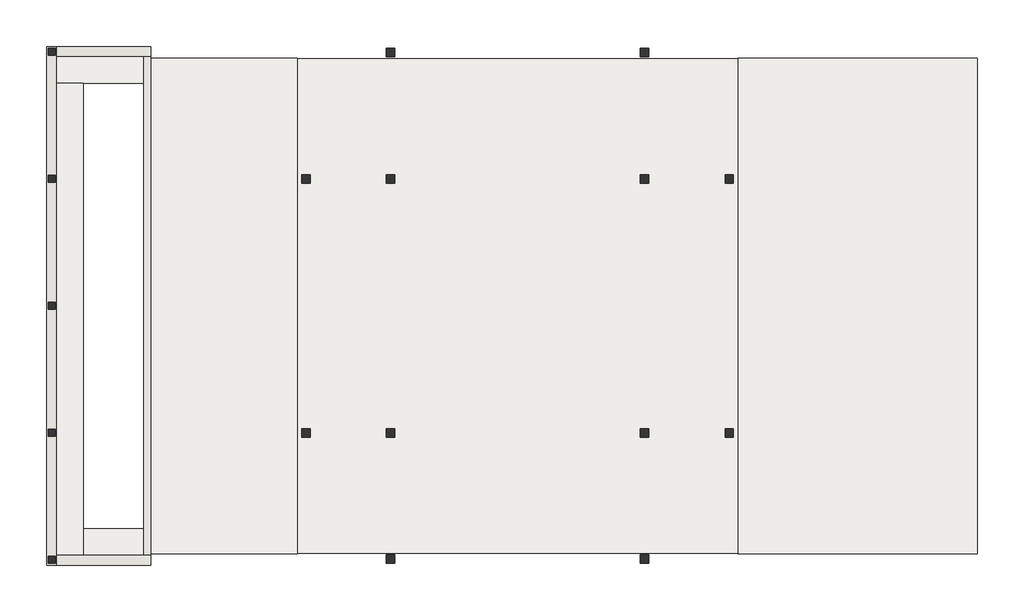
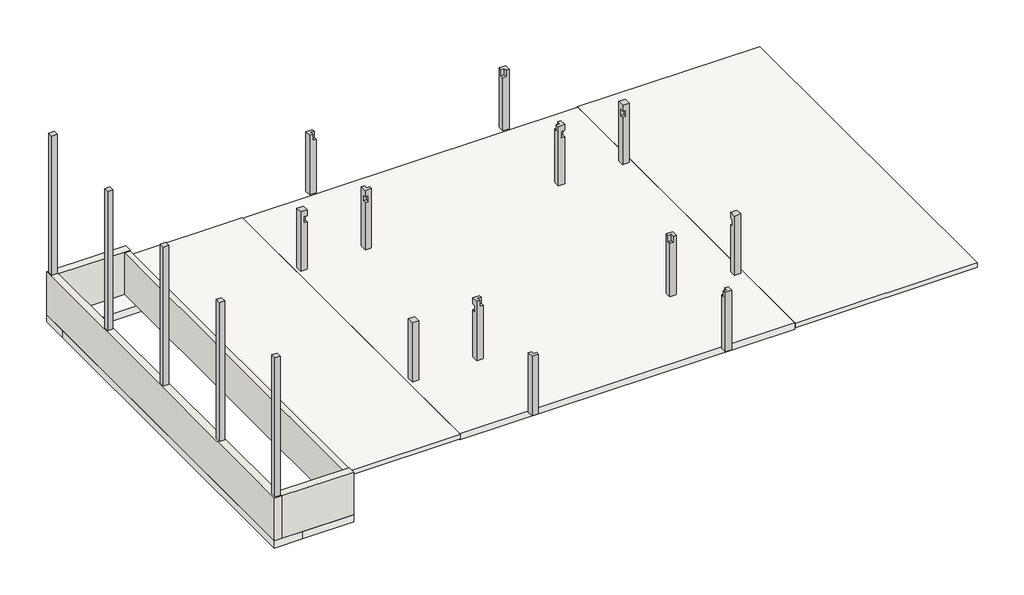
# One storey: 17 columns, 4 walls, 3 footings, 3 slabs.
"""IFC4 building model written with IfcOpenShell, lengths in millimetres."""

import ifcopenshell
import ifcopenshell.guid

model = None  # the IFC model being written
_history = None  # IfcOwnerHistory: only IFC2X3 demands one
_inside = {}  # id of a spatial element -> (the spatial element, [elements in it])
_under = {}  # id of a project, library or spatial element -> (it, [spatial elements below it])
_declared = {}  # id of a project -> (the project, [libraries it declares])
_typed = {}  # id of a type object -> (the type object, [elements of that type])
_made_of = {}  # id of a material, layer set ... -> (it, [elements and type objects made of it])


def new_model(schema):
    """Start an empty IFC model of exactly this schema.

    Asked for "IFC4X3", IfcOpenShell would pick the latest addendum, in which some entities
    have other attributes; the version numbers below select the first issue.
    IFC2X3 requires an IfcOwnerHistory on every rooted entity: one is made here for all.
    """
    global model, _history
    if schema == "IFC4X3":
        model = ifcopenshell.file(schema_version=(4, 3, 0, 0))
    else:
        model = ifcopenshell.file(schema=schema)
    _inside.clear()
    _under.clear()
    _declared.clear()
    _typed.clear()
    _made_of.clear()
    _history = None
    if model.schema == "IFC2X3":
        org = make("IfcOrganization", Name="unknown")
        user = make(
            "IfcPersonAndOrganization",
            ThePerson=make("IfcPerson", FamilyName="unknown"),
            TheOrganization=org,
        )
        app = make(
            "IfcApplication",
            ApplicationDeveloper=org,
            Version="unknown",
            ApplicationFullName="unknown",
            ApplicationIdentifier="unknown",
        )
        _history = make(
            "IfcOwnerHistory",
            OwningUser=user,
            OwningApplication=app,
            ChangeAction="ADDED",
            CreationDate=0,
        )
    return model


def make(cls, **values):
    """One entity of the class cls with the attributes given. An attribute that is None is left unset."""
    return model.create_entity(
        cls, **{name: value for name, value in values.items() if value is not None}
    )


def rooted(cls, **values):
    """An entity with a GlobalId (a new one), such as an element, a storey or a relation."""
    return make(cls, GlobalId=ifcopenshell.guid.new(), OwnerHistory=_history, **values)


def si_unit(unit_type, name, prefix=None):
    """IfcSIUnit, for example si_unit("LENGTHUNIT", "METRE", prefix="MILLI")."""
    return make("IfcSIUnit", UnitType=unit_type, Prefix=prefix, Name=name)


def assignment(units):
    """IfcUnitAssignment: the units of a project."""
    return None if units is None else make("IfcUnitAssignment", Units=units)


def point(xyz):
    """IfcCartesianPoint."""
    return None if xyz is None else make("IfcCartesianPoint", Coordinates=xyz)


def direction(xyz):
    """IfcDirection."""
    return None if xyz is None else make("IfcDirection", DirectionRatios=xyz)


def frame(location, z_axis=None, x_axis=None):
    """IfcAxis2Placement3D, a coordinate frame: its origin and axes. An axis left out is left unset."""
    return make(
        "IfcAxis2Placement3D",
        Location=point(location),
        Axis=direction(z_axis),
        RefDirection=direction(x_axis),
    )


def origin():
    """The frame at (0, 0, 0) with its axes left unset."""
    return frame((0.0, 0.0, 0.0))


def origin_with_axes():
    """The frame at (0, 0, 0) with the z axis (0, 0, 1) and the x axis (1, 0, 0) written out."""
    return frame((0.0, 0.0, 0.0), z_axis=(0.0, 0.0, 1.0), x_axis=(1.0, 0.0, 0.0))


def place(relative_to, where):
    """IfcLocalPlacement: puts the frame where relative to a parent placement (None: the world)."""
    return make(
        "IfcLocalPlacement", PlacementRelTo=relative_to, RelativePlacement=where
    )


def context(
    kind, dimensions, precision=None, world=None, true_north=None, identifier=None
):
    """IfcGeometricRepresentationContext, for example the 3D "Model" context."""
    return make(
        "IfcGeometricRepresentationContext",
        ContextIdentifier=identifier,
        ContextType=kind,
        CoordinateSpaceDimension=dimensions,
        Precision=precision,
        WorldCoordinateSystem=world,
        TrueNorth=true_north,
    )


def project(units=None, contexts=None):
    """IfcProject with its units and contexts."""
    return rooted(
        "IfcProject",
        Name="project",
        RepresentationContexts=contexts,
        UnitsInContext=assignment(units),
    )


def spatial(cls, under=None, at=None, **own):
    """A site, building, storey or space (cls), placed at a placement, below another one or the project."""
    s = rooted(cls, ObjectPlacement=at, **own)
    if under is not None:
        _under.setdefault(under.id(), (under, []))[1].append(s)
    return s


def polyline(points):
    """IfcPolyline through the points."""
    return make("IfcPolyline", Points=[point(p) for p in points])


def outline(outer, holes=None, kind="AREA"):
    """IfcArbitraryClosedProfileDef: a profile drawn as a closed curve; with holes, ...WithVoids."""
    if holes is None:
        return make("IfcArbitraryClosedProfileDef", ProfileType=kind, OuterCurve=outer)
    return make(
        "IfcArbitraryProfileDefWithVoids",
        ProfileType=kind,
        OuterCurve=outer,
        InnerCurves=holes,
    )


def extrude(swept, where, along, depth):
    """IfcExtrudedAreaSolid: the profile swept, set in the frame where, extruded along a direction by depth."""
    return make(
        "IfcExtrudedAreaSolid",
        SweptArea=swept,
        Position=where,
        ExtrudedDirection=direction(along),
        Depth=depth,
    )


def faces_of(points, faces, orient=None, outer=None):
    """IfcFace entities. A face is a list of loops; a loop is a list of indices into points, from 0.

    orient and outer hold one flag for each loop. By default every Orientation is true, the
    first loop of a face is its IfcFaceOuterBound and the others are IfcFaceBound.
    """
    made = []
    for i, loops in enumerate(faces):
        bounds = []
        for j, loop in enumerate(loops):
            is_outer = j == 0 if outer is None else outer[i][j]
            bounds.append(
                make(
                    "IfcFaceOuterBound" if is_outer else "IfcFaceBound",
                    Bound=make("IfcPolyLoop", Polygon=[points[k] for k in loop]),
                    Orientation=True if orient is None else orient[i][j],
                )
            )
        made.append(make("IfcFace", Bounds=bounds))
    return made


def faceted_brep(points, faces, orient=None, outer=None, voids=None):
    """IfcFacetedBrep: a solid bounded by flat faces; with voids (closed shells), ...WithVoids."""
    shared = [point(p) for p in points]
    hull = make("IfcClosedShell", CfsFaces=faces_of(shared, faces, orient, outer))
    if voids is None:
        return make("IfcFacetedBrep", Outer=hull)
    return make(
        "IfcFacetedBrepWithVoids",
        Outer=hull,
        Voids=[
            make(cls, CfsFaces=faces_of(shared, fs, o, b)) for cls, fs, o, b in voids
        ],
    )


def shape(context_of_items, identifier, shape_type, items):
    """IfcShapeRepresentation: the items that make up one representation, for example the "Body"."""
    return make(
        "IfcShapeRepresentation",
        ContextOfItems=context_of_items,
        RepresentationIdentifier=identifier,
        RepresentationType=shape_type,
        Items=items,
    )


def made_of(thing, what):
    """Note that an element or type object is made of a material, layer set ...; save() writes the relation."""
    if what is not None:
        _made_of.setdefault(what.id(), (what, []))[1].append(thing)
    return thing


def element(
    cls,
    number,
    at=None,
    inside=None,
    cuts=None,
    type_object=None,
    material=None,
    context=None,
    identifier="Body",
    shape_type=None,
    held_by="IfcProductDefinitionShape",
    body=None,
    shapes=None,
    **own,
):
    """One element of the class cls, such as IfcWall. Its Tag is "e" and its number.

    at: its placement. inside: the storey or other place that contains it. cuts: it is an
    opening in that element (IfcRelVoidsElement). A single representation is given by context,
    identifier, shape_type and body (its items); several are given by shapes. held_by: the class
    of the entity that holds the representations. save() writes the other relations.
    """
    e = rooted(cls, Tag="e%d" % number, ObjectPlacement=at, **own)
    if body is not None:
        shapes = [shape(context, identifier, shape_type, body)]
    if shapes is not None:
        e.Representation = make(held_by, Representations=shapes)
    if inside is not None:
        _inside.setdefault(inside.id(), (inside, []))[1].append(e)
    if cuts is not None:
        rooted(
            "IfcRelVoidsElement", RelatingBuildingElement=cuts, RelatedOpeningElement=e
        )
    if type_object is not None:
        _typed.setdefault(type_object.id(), (type_object, []))[1].append(e)
    return made_of(e, material)


def aggregate(whole, parts):
    """IfcRelAggregates: a whole, such as a stair, and the parts it consists of."""
    return rooted("IfcRelAggregates", RelatingObject=whole, RelatedObjects=parts)


def save(model, path):
    """Write the relations noted so far, then the file.

    IfcRelAggregates (storeys below a building ...), IfcRelContainedInSpatialStructure (elements
    in a storey), IfcRelDefinesByType, IfcRelAssociatesMaterial and IfcRelDeclares: one each for
    every whole, place, type object, material and project.
    """
    for whole, parts in _under.values():
        aggregate(whole, parts)
    for where, things in _inside.values():
        rooted(
            "IfcRelContainedInSpatialStructure",
            RelatedElements=things,
            RelatingStructure=where,
        )
    for kind, things in _typed.values():
        rooted("IfcRelDefinesByType", RelatedObjects=things, RelatingType=kind)
    for what, things in _made_of.values():
        rooted("IfcRelAssociatesMaterial", RelatedObjects=things, RelatingMaterial=what)
    for by, libraries in _declared.values():
        rooted("IfcRelDeclares", RelatingContext=by, RelatedDefinitions=libraries)
    model.write(path)


model = new_model("IFC4")

# Units and contexts
model_context = context("Model", 3, world=origin())
ifc_project = project(units=[si_unit("LENGTHUNIT", "METRE", prefix="MILLI")], contexts=[model_context])

# Site, building, storey
site = spatial("IfcSite", under=ifc_project)
building = spatial("IfcBuilding", under=site)
storey = spatial("IfcBuildingStorey", under=building, Name="E-ACCESO", Elevation=0.0)

# Columns
placement = place(None, origin())
element("IfcColumn", 1, ObjectType="Hormigón-Cuadrado-Pilar : PILAR 25X25", at=placement, inside=storey, context=model_context, shape_type="SweptSolid", body=[
    extrude(outline(polyline([(-32875.0, -4375.0), (-32875.0, -4625.0), (-33125.0, -4625.0), (-33125.0, -4375.0), (-32875.0, -4375.0)])), origin_with_axes(), (0.0, 0.0, 1.0), 6850.0),
])
element("IfcColumn", 2, ObjectType="Hormigón-Cuadrado-Pilar : PILAR 25X25", at=placement, inside=storey, context=model_context, shape_type="SweptSolid", body=[
    extrude(outline(polyline([(-32875.0, -8875.0), (-32875.0, -9125.0), (-33125.0, -9125.0), (-33125.0, -8875.0), (-32875.0, -8875.0)])), origin_with_axes(), (0.0, 0.0, 1.0), 6850.0),
])
element("IfcColumn", 3, ObjectType="Hormigón-Cuadrado-Pilar : PILAR 25X25", at=placement, inside=storey, context=model_context, shape_type="SweptSolid", body=[
    extrude(outline(polyline([(-32875.0, -13375.0), (-32875.0, -13625.0), (-33125.0, -13625.0), (-33125.0, -13375.0), (-32875.0, -13375.0)])), origin_with_axes(), (0.0, 0.0, 1.0), 6850.0),
])
element("IfcColumn", 4, ObjectType="Hormigón-Cuadrado-Pilar : PILAR 25X25", at=placement, inside=storey, context=model_context, shape_type="SweptSolid", body=[
    extrude(outline(polyline([(-32875.0, -17875.0), (-32875.0, -18125.0), (-33125.0, -18125.0), (-33125.0, -17875.0), (-32875.0, -17875.0)])), origin_with_axes(), (0.0, 0.0, 1.0), 6850.0),
])
element("IfcColumn", 5, ObjectType="Hormigón-Cuadrado-Pilar : PILAR 25X25", at=placement, inside=storey, context=model_context, shape_type="SweptSolid", body=[
    extrude(outline(polyline([(-32875.0, 125.0), (-32875.0, -125.0), (-33125.0, -125.0), (-33125.0, 125.0), (-32875.0, 125.0)])), origin_with_axes(), (0.0, 0.0, 1.0), 6850.0),
])
element("IfcColumn", 6, ObjectType="Hormigón-Cuadrado-Pilar : PILAR 30X30", at=placement, inside=storey, context=model_context, shape_type="Brep", body=[
    faceted_brep([(-23850.0, -4350.0, -200.0), (-23850.0, -4650.0, -200.0), (-24150.0, -4650.0, -200.0), (-24150.0, -4350.0, -200.0), (-23850.0, -4350.0, 2730.0), (-23850.0, -4650.0, 2730.0), (-23850.0, -4650.0, 2430.0), (-23850.0, -4500.0, 2430.0), (-23850.0, -4500.0, 2130.0), (-23850.0, -4650.0, 2130.0), (-24000.0, -4650.0, 2130.0), (-24000.0, -4650.0, 2430.0), (-24150.0, -4650.0, 2730.0), (-24150.0, -4350.0, 2730.0), (-24000.0, -4500.0, 2130.0), (-24000.0, -4500.0, 2430.0)], [[[0, 1, 2, 3]], [[1, 0, 4, 5, 6, 7, 8, 9]], [[2, 1, 9, 10, 11, 6, 5, 12]], [[3, 2, 12, 13]], [[0, 3, 13, 4]], [[5, 4, 13, 12]], [[8, 14, 10, 9]], [[11, 15, 7, 6]], [[14, 15, 11, 10]], [[15, 14, 8, 7]]]),
])
element("IfcColumn", 7, ObjectType="Hormigón-Cuadrado-Pilar : PILAR 30X30", at=placement, inside=storey, context=model_context, shape_type="Brep", body=[
    faceted_brep([(-20850.0, -4350.0, -200.0), (-20850.0, -4650.0, -200.0), (-21150.0, -4650.0, -200.0), (-21150.0, -4350.0, -200.0), (-20850.0, -4350.0, 2430.0), (-20850.0, -4500.0, 2430.0), (-20850.0, -4500.0, 2730.0), (-20850.0, -4650.0, 2730.0), (-21150.0, -4650.0, 2730.0), (-21150.0, -4650.0, 2430.0), (-21000.0, -4650.0, 2430.0), (-21000.0, -4650.0, 2130.0), (-21150.0, -4650.0, 2130.0), (-21150.0, -4500.0, 2130.0), (-21150.0, -4500.0, 2430.0), (-21150.0, -4350.0, 2730.0), (-21000.0, -4350.0, 2730.0), (-21000.0, -4350.0, 2430.0), (-21000.0, -4500.0, 2730.0), (-21000.0, -4500.0, 2430.0), (-21000.0, -4500.0, 2130.0), (-21000.0, -4500.0, 2430.0)], [[[0, 1, 2, 3]], [[1, 0, 4, 5, 6, 7]], [[2, 1, 7, 8, 9, 10, 11, 12]], [[3, 2, 12, 13, 14, 9, 8, 15]], [[0, 3, 15, 16, 17, 4]], [[8, 7, 6, 18, 16, 15]], [[19, 5, 4, 17]], [[18, 19, 17, 16]], [[19, 18, 6, 5]], [[20, 13, 12, 11]], [[21, 10, 9, 14]], [[21, 20, 11, 10]], [[20, 21, 14, 13]]]),
])
element("IfcColumn", 8, ObjectType="Hormigón-Cuadrado-Pilar : PILAR 30X30", at=placement, inside=storey, context=model_context, shape_type="Brep", body=[
    faceted_brep([(-11850.0, -4350.0, -200.0), (-11850.0, -4650.0, -200.0), (-12150.0, -4650.0, -200.0), (-12150.0, -4350.0, -200.0), (-11850.0, -4350.0, 2730.0), (-11850.0, -4650.0, 2730.0), (-11850.0, -4650.0, 2430.0), (-11850.0, -4500.0, 2430.0), (-11850.0, -4500.0, 2130.0), (-11850.0, -4650.0, 2130.0), (-12000.0, -4650.0, 2130.0), (-12000.0, -4650.0, 2430.0), (-12150.0, -4650.0, 2730.0), (-12150.0, -4500.0, 2730.0), (-12150.0, -4500.0, 2430.0), (-12150.0, -4350.0, 2430.0), (-12000.0, -4350.0, 2430.0), (-12000.0, -4350.0, 2730.0), (-12000.0, -4500.0, 2730.0), (-12000.0, -4500.0, 2430.0), (-12000.0, -4500.0, 2130.0), (-12000.0, -4500.0, 2430.0)], [[[0, 1, 2, 3]], [[1, 0, 4, 5, 6, 7, 8, 9]], [[2, 1, 9, 10, 11, 6, 5, 12]], [[3, 2, 12, 13, 14, 15]], [[0, 3, 15, 16, 17, 4]], [[5, 4, 17, 18, 13, 12]], [[14, 19, 16, 15]], [[19, 18, 17, 16]], [[18, 19, 14, 13]], [[8, 20, 10, 9]], [[11, 21, 7, 6]], [[20, 21, 11, 10]], [[21, 20, 8, 7]]]),
])
element("IfcColumn", 9, ObjectType="Hormigón-Cuadrado-Pilar : PILAR 30X30", at=placement, inside=storey, context=model_context, shape_type="Brep", body=[
    faceted_brep([(-8850.0, -4350.0, -200.0), (-8850.0, -4650.0, -200.0), (-9150.0, -4650.0, -200.0), (-9150.0, -4350.0, -200.0), (-8850.0, -4350.0, 2730.0), (-8850.0, -4650.0, 2730.0), (-9150.0, -4650.0, 2730.0), (-9150.0, -4650.0, 2430.0), (-9000.0, -4650.0, 2430.0), (-9000.0, -4650.0, 2130.0), (-9150.0, -4650.0, 2130.0), (-9150.0, -4500.0, 2130.0), (-9150.0, -4500.0, 2430.0), (-9150.0, -4350.0, 2730.0), (-9000.0, -4500.0, 2130.0), (-9000.0, -4500.0, 2430.0)], [[[0, 1, 2, 3]], [[1, 0, 4, 5]], [[2, 1, 5, 6, 7, 8, 9, 10]], [[3, 2, 10, 11, 12, 7, 6, 13]], [[0, 3, 13, 4]], [[5, 4, 13, 6]], [[14, 11, 10, 9]], [[15, 8, 7, 12]], [[15, 14, 9, 8]], [[14, 15, 12, 11]]]),
])
element("IfcColumn", 10, ObjectType="Hormigón-Cuadrado-Pilar : PILAR 30X30", at=placement, inside=storey, context=model_context, shape_type="Brep", body=[
    faceted_brep([(-8850.0, -13350.0, -200.0), (-8850.0, -13650.0, -200.0), (-9150.0, -13650.0, -200.0), (-9150.0, -13350.0, -200.0), (-8850.0, -13350.0, 2730.0), (-8850.0, -13650.0, 2730.0), (-9150.0, -13650.0, 2730.0), (-9150.0, -13350.0, 2730.0), (-9150.0, -13350.0, 2430.0), (-9150.0, -13500.0, 2430.0), (-9150.0, -13500.0, 2130.0), (-9150.0, -13350.0, 2130.0), (-9000.0, -13350.0, 2130.0), (-9000.0, -13350.0, 2430.0), (-9000.0, -13500.0, 2130.0), (-9000.0, -13500.0, 2430.0)], [[[0, 1, 2, 3]], [[1, 0, 4, 5]], [[2, 1, 5, 6]], [[3, 2, 6, 7, 8, 9, 10, 11]], [[0, 3, 11, 12, 13, 8, 7, 4]], [[5, 4, 7, 6]], [[10, 14, 12, 11]], [[13, 15, 9, 8]], [[14, 15, 13, 12]], [[15, 14, 10, 9]]]),
])
element("IfcColumn", 11, ObjectType="Hormigón-Cuadrado-Pilar : PILAR 30X30", at=placement, inside=storey, context=model_context, shape_type="Brep", body=[
    faceted_brep([(-11850.0, -13350.0, -200.0), (-11850.0, -13650.0, -200.0), (-12150.0, -13650.0, -200.0), (-12150.0, -13350.0, -200.0), (-11850.0, -13350.0, 2130.0), (-11850.0, -13500.0, 2130.0), (-11850.0, -13500.0, 2430.0), (-11850.0, -13350.0, 2430.0), (-11850.0, -13350.0, 2730.0), (-11850.0, -13650.0, 2730.0), (-12000.0, -13650.0, 2730.0), (-12000.0, -13650.0, 2430.0), (-12150.0, -13650.0, 2430.0), (-12150.0, -13500.0, 2430.0), (-12150.0, -13500.0, 2730.0), (-12150.0, -13350.0, 2730.0), (-12000.0, -13350.0, 2430.0), (-12000.0, -13350.0, 2130.0), (-12000.0, -13500.0, 2730.0), (-12000.0, -13500.0, 2430.0), (-12000.0, -13500.0, 2130.0), (-12000.0, -13500.0, 2430.0)], [[[0, 1, 2, 3]], [[1, 0, 4, 5, 6, 7, 8, 9]], [[2, 1, 9, 10, 11, 12]], [[3, 2, 12, 13, 14, 15]], [[0, 3, 15, 8, 7, 16, 17, 4]], [[9, 8, 15, 14, 18, 10]], [[19, 13, 12, 11]], [[18, 19, 11, 10]], [[19, 18, 14, 13]], [[17, 20, 5, 4]], [[6, 21, 16, 7]], [[20, 21, 6, 5]], [[21, 20, 17, 16]]]),
])
element("IfcColumn", 12, ObjectType="Hormigón-Cuadrado-Pilar : PILAR 30X30", at=placement, inside=storey, context=model_context, shape_type="Brep", body=[
    faceted_brep([(-20850.0, -13350.0, -200.0), (-20850.0, -13650.0, -200.0), (-21150.0, -13650.0, -200.0), (-21150.0, -13350.0, -200.0), (-20850.0, -13350.0, 2730.0), (-20850.0, -13500.0, 2730.0), (-20850.0, -13500.0, 2430.0), (-20850.0, -13650.0, 2430.0), (-21000.0, -13650.0, 2430.0), (-21000.0, -13650.0, 2730.0), (-21150.0, -13650.0, 2730.0), (-21150.0, -13350.0, 2730.0), (-21150.0, -13350.0, 2430.0), (-21150.0, -13500.0, 2430.0), (-21150.0, -13500.0, 2130.0), (-21150.0, -13350.0, 2130.0), (-21000.0, -13350.0, 2130.0), (-21000.0, -13350.0, 2430.0), (-21000.0, -13500.0, 2730.0), (-21000.0, -13500.0, 2430.0), (-21000.0, -13500.0, 2130.0), (-21000.0, -13500.0, 2430.0)], [[[0, 1, 2, 3]], [[1, 0, 4, 5, 6, 7]], [[2, 1, 7, 8, 9, 10]], [[3, 2, 10, 11, 12, 13, 14, 15]], [[0, 3, 15, 16, 17, 12, 11, 4]], [[11, 10, 9, 18, 5, 4]], [[6, 19, 8, 7]], [[19, 18, 9, 8]], [[18, 19, 6, 5]], [[14, 20, 16, 15]], [[17, 21, 13, 12]], [[20, 21, 17, 16]], [[21, 20, 14, 13]]]),
])
element("IfcColumn", 13, ObjectType="Hormigón-Cuadrado-Pilar : PILAR 30X30", at=placement, inside=storey, context=model_context, shape_type="Brep", body=[
    faceted_brep([(-23850.0, -13350.0, -200.0), (-23850.0, -13650.0, -200.0), (-24150.0, -13650.0, -200.0), (-24150.0, -13350.0, -200.0), (-23850.0, -13350.0, 2130.0), (-23850.0, -13500.0, 2130.0), (-23850.0, -13500.0, 2430.0), (-23850.0, -13350.0, 2430.0), (-23850.0, -13350.0, 2730.0), (-23850.0, -13650.0, 2730.0), (-24150.0, -13650.0, 2730.0), (-24150.0, -13350.0, 2730.0), (-24000.0, -13350.0, 2430.0), (-24000.0, -13350.0, 2130.0), (-24000.0, -13500.0, 2130.0), (-24000.0, -13500.0, 2430.0)], [[[0, 1, 2, 3]], [[1, 0, 4, 5, 6, 7, 8, 9]], [[2, 1, 9, 10]], [[3, 2, 10, 11]], [[0, 3, 11, 8, 7, 12, 13, 4]], [[9, 8, 11, 10]], [[13, 14, 5, 4]], [[6, 15, 12, 7]], [[14, 15, 6, 5]], [[15, 14, 13, 12]]]),
])
element("IfcColumn", 14, ObjectType="Hormigón-Cuadrado-Pilar : PILAR 30X30", at=placement, inside=storey, context=model_context, shape_type="Brep", body=[
    faceted_brep([(-20850.0, -17825.0, -200.0), (-20850.0, -18125.0, -200.0), (-21150.0, -18125.0, -200.0), (-21150.0, -17825.0, -200.0), (-20850.0, -17825.0, 2430.0), (-20850.0, -17975.0, 2430.0), (-20850.0, -17975.0, 2730.0), (-20850.0, -18125.0, 2730.0), (-21150.0, -18125.0, 2730.0), (-21150.0, -17825.0, 2730.0), (-21000.0, -17825.0, 2730.0), (-21000.0, -17825.0, 2430.0), (-21000.0, -17975.0, 2730.0), (-21000.0, -17975.0, 2430.0)], [[[0, 1, 2, 3]], [[1, 0, 4, 5, 6, 7]], [[2, 1, 7, 8]], [[3, 2, 8, 9]], [[0, 3, 9, 10, 11, 4]], [[8, 7, 6, 12, 10, 9]], [[11, 13, 5, 4]], [[13, 12, 6, 5]], [[12, 13, 11, 10]]]),
])
element("IfcColumn", 15, ObjectType="Hormigón-Cuadrado-Pilar : PILAR 30X30", at=placement, inside=storey, context=model_context, shape_type="Brep", body=[
    faceted_brep([(-20850.0, 125.0, -200.0), (-20850.0, -175.0, -200.0), (-21150.0, -175.0, -200.0), (-21150.0, 125.0, -200.0), (-20850.0, 125.0, 2730.0), (-20850.0, -25.0, 2730.0), (-20850.0, -25.0, 2430.0), (-20850.0, -175.0, 2430.0), (-21150.0, 125.0, 2730.0), (-21150.0, -175.0, 2730.0), (-21000.0, -175.0, 2430.0), (-21000.0, -175.0, 2730.0), (-21000.0, -25.0, 2730.0), (-21000.0, -25.0, 2430.0)], [[[0, 1, 2, 3]], [[1, 0, 4, 5, 6, 7]], [[0, 3, 8, 4]], [[3, 2, 9, 8]], [[2, 1, 7, 10, 11, 9]], [[4, 8, 9, 11, 12, 5]], [[6, 13, 10, 7]], [[13, 12, 11, 10]], [[12, 13, 6, 5]]]),
])
element("IfcColumn", 16, ObjectType="Hormigón-Cuadrado-Pilar : PILAR 30X30", at=placement, inside=storey, context=model_context, shape_type="Brep", body=[
    faceted_brep([(-12150.0, -18125.0, -200.0), (-12150.0, -17825.0, -200.0), (-11850.0, -17825.0, -200.0), (-11850.0, -18125.0, -200.0), (-12150.0, -18125.0, 2730.0), (-12150.0, -17975.0, 2730.0), (-12150.0, -17975.0, 2430.0), (-12150.0, -17825.0, 2430.0), (-11850.0, -18125.0, 2730.0), (-11850.0, -17825.0, 2730.0), (-12000.0, -17825.0, 2430.0), (-12000.0, -17825.0, 2730.0), (-12000.0, -17975.0, 2730.0), (-12000.0, -17975.0, 2430.0)], [[[0, 1, 2, 3]], [[1, 0, 4, 5, 6, 7]], [[0, 3, 8, 4]], [[3, 2, 9, 8]], [[2, 1, 7, 10, 11, 9]], [[4, 8, 9, 11, 12, 5]], [[6, 13, 10, 7]], [[13, 12, 11, 10]], [[12, 13, 6, 5]]]),
])
element("IfcColumn", 17, ObjectType="Hormigón-Cuadrado-Pilar : PILAR 30X30", at=placement, inside=storey, context=model_context, shape_type="Brep", body=[
    faceted_brep([(-12150.0, -175.0, -200.0), (-12150.0, 125.0, -200.0), (-11850.0, 125.0, -200.0), (-11850.0, -175.0, -200.0), (-12150.0, -175.0, 2430.0), (-12150.0, -25.0, 2430.0), (-12150.0, -25.0, 2730.0), (-12150.0, 125.0, 2730.0), (-11850.0, 125.0, 2730.0), (-11850.0, -175.0, 2730.0), (-12000.0, -175.0, 2730.0), (-12000.0, -175.0, 2430.0), (-12000.0, -25.0, 2730.0), (-12000.0, -25.0, 2430.0)], [[[0, 1, 2, 3]], [[1, 0, 4, 5, 6, 7]], [[2, 1, 7, 8]], [[3, 2, 8, 9]], [[0, 3, 9, 10, 11, 4]], [[8, 7, 6, 12, 10, 9]], [[11, 13, 5, 4]], [[13, 12, 6, 5]], [[12, 13, 11, 10]]]),
])

# Footings
element("IfcFooting", 18, ObjectType="CIMENT MURO PISCINA_PABLO", at=placement, inside=storey, context=model_context, shape_type="Brep", body=[
    faceted_brep([(-31890.0, -18190.0, -2100.0), (-31890.0, -16890.0, -2100.0), (-31890.0, -1110.0, -2100.0), (-33190.0, -1110.0, -2100.0), (-33190.0, -18190.0, -2100.0), (-32840.0, -18190.0, -2100.0), (-33190.0, -18190.0, -2450.0), (-33190.0, -1110.0, -2450.0), (-31890.0, -18190.0, -2450.0), (-31890.0, -1110.0, -2450.0), (-31890.0, -16890.0, -2450.0)], [[[0, 1, 2, 3, 4, 5]], [[6, 4, 3, 7]], [[8, 6, 7, 9, 10]], [[0, 8, 10, 9, 2, 1]], [[3, 2, 9, 7]], [[0, 5, 4, 6, 8]]]),
])
element("IfcFooting", 19, ObjectType="CIMENT MURO PISCINA_PABLO", at=placement, inside=storey, context=model_context, shape_type="Brep", body=[
    faceted_brep([(-29500.0, 190.0, -2100.0), (-29500.0, -1110.0, -2100.0), (-29500.0, -1110.0, -2450.0), (-29500.0, 190.0, -2450.0), (-33190.0, -1110.0, -2100.0), (-31890.0, -1110.0, -2100.0), (-33190.0, 190.0, -2100.0), (-33190.0, 190.0, -2450.0), (-33190.0, -1110.0, -2450.0), (-31890.0, -1110.0, -2450.0)], [[[0, 1, 2, 3]], [[4, 5, 1, 0, 6]], [[7, 6, 0, 3]], [[8, 7, 3, 2, 9]], [[4, 8, 9, 2, 1, 5]], [[4, 6, 7, 8]]]),
])
element("IfcFooting", 20, ObjectType="CIMENT MURO PISCINA_PABLO", at=placement, inside=storey, context=model_context, shape_type="SweptSolid", body=[
    extrude(outline(polyline([(-29500.0, -16890.0), (-29500.0, -18190.0), (-31890.0, -18190.0), (-31890.0, -16890.0), (-29500.0, -16890.0)])), frame((0.0, 0.0, -2450.0), z_axis=(0.0, 0.0, 1.0), x_axis=(1.0, 0.0, 0.0)), (0.0, 0.0, 1.0), 350.0),
])

# Slabs
element("IfcSlab", 21, ObjectType="FORJADO 1_PABLO", at=placement, inside=storey, context=model_context, shape_type="SweptSolid", body=[
    extrude(outline(polyline([(-24300.0, -237.5), (-8700.0, -237.5), (-8700.0, -17762.5), (-24300.0, -17762.5), (-24300.0, -237.5)])), frame((0.0, 0.0, -500.0), z_axis=(0.0, 0.0, 1.0), x_axis=(1.0, 0.0, 0.0)), (0.0, 0.0, 1.0), 300.0),
])
element("IfcSlab", 22, ObjectType="FORJ HORM EXT_PABLO", at=placement, inside=storey, context=model_context, shape_type="SweptSolid", body=[
    extrude(outline(polyline([(-8700.0, -220.0), (-205.0, -220.0), (-205.0, -17780.0), (-8700.0, -17780.0), (-8700.0, -220.0)])), frame((0.0, 0.0, -425.0), z_axis=(0.0, 0.0, 1.0), x_axis=(1.0, 0.0, 0.0)), (0.0, 0.0, 1.0), 225.0),
])
element("IfcSlab", 23, ObjectType="FORJ HORM EXT_PABLO", at=placement, inside=storey, context=model_context, shape_type="SweptSolid", body=[
    extrude(outline(polyline([(-29500.0, -220.0), (-24300.0, -220.0), (-24300.0, -17780.0), (-29500.0, -17780.0), (-29500.0, -220.0)])), frame((0.0, 0.0, -425.0), z_axis=(0.0, 0.0, 1.0), x_axis=(1.0, 0.0, 0.0)), (0.0, 0.0, 1.0), 225.0),
])

# Walls
element("IfcWall", 24, ObjectType="MURO 1 HORM VASO PISCINA_PABLO", at=placement, inside=storey, context=model_context, shape_type="Brep", body=[
    faceted_brep([(-32840.0, -18190.0, -2100.0), (-32840.0, -17840.0, -2100.0), (-32840.0, -160.0, -2100.0), (-32840.0, 190.0, -2100.0), (-32840.0, 190.0, 0.0), (-32840.0, -160.0, 0.0), (-32840.0, -17840.0, 0.0), (-32840.0, -18190.0, 0.0), (-33190.0, -18190.0, -2100.0), (-33190.0, -18190.0, 0.0), (-33190.0, 190.0, 0.0), (-33190.0, 190.0, -2100.0), (-33190.0, -1110.0, -2100.0)], [[[0, 1, 2, 3, 4, 5, 6, 7]], [[8, 9, 10, 11, 12]], [[3, 2, 1, 0, 8, 12, 11]], [[7, 6, 5, 4, 10, 9]], [[0, 7, 9, 8]], [[4, 3, 11, 10]]]),
])
element("IfcWall", 25, ObjectType="MURO 2 HORM VASO PISCINA_PABLO", at=placement, inside=storey, context=model_context, shape_type="Brep", body=[
    faceted_brep([(-29500.0, -17840.0, -2100.0), (-29500.0, -160.0, -2100.0), (-29500.0, -160.0, -50.0), (-29500.0, -17840.0, -50.0), (-29750.0, -17840.0, -2100.0), (-29750.0, -17840.0, -1850.0), (-29750.0, -17840.0, -50.0), (-29750.0, -160.0, -50.0), (-29750.0, -160.0, -1850.0), (-29750.0, -160.0, -2100.0)], [[[0, 1, 2, 3]], [[4, 5, 6, 7, 8, 9]], [[1, 0, 4, 9]], [[3, 2, 7, 6]], [[0, 3, 6, 5, 4]], [[2, 1, 9, 8, 7]]]),
])
element("IfcWall", 26, ObjectType="MURO 1 HORM VASO PISCINA_PABLO", at=placement, inside=storey, context=model_context, shape_type="Brep", body=[
    faceted_brep([(-32840.0, -18190.0, -2100.0), (-29500.0, -18190.0, -2100.0), (-29500.0, -18190.0, -1500.0), (-29500.0, -18190.0, -900.0), (-29500.0, -18190.0, 0.0), (-32840.0, -18190.0, 0.0), (-32840.0, -17840.0, -2100.0), (-32840.0, -17840.0, -1850.0), (-32840.0, -17840.0, 0.0), (-29500.0, -17840.0, 0.0), (-29500.0, -17840.0, -50.0), (-29500.0, -17840.0, -2100.0), (-29750.0, -17840.0, -2100.0)], [[[0, 1, 2, 3, 4, 5]], [[6, 7, 8, 9, 10, 11, 12]], [[1, 0, 6, 12, 11]], [[5, 4, 9, 8]], [[0, 5, 8, 7, 6]], [[4, 3, 2, 1, 11, 10, 9]]]),
])
element("IfcWall", 27, ObjectType="MURO 1 HORM VASO PISCINA_PABLO", at=placement, inside=storey, context=model_context, shape_type="Brep", body=[
    faceted_brep([(-32840.0, -160.0, -2100.0), (-29750.0, -160.0, -2100.0), (-29500.0, -160.0, -2100.0), (-29500.0, -160.0, -50.0), (-29500.0, -160.0, 0.0), (-32840.0, -160.0, 0.0), (-32840.0, -160.0, -1850.0), (-32840.0, 190.0, -2100.0), (-32840.0, 190.0, 0.0), (-29500.0, 190.0, 0.0), (-29500.0, 190.0, -900.0), (-29500.0, 190.0, -1500.0), (-29500.0, 190.0, -2100.0)], [[[0, 1, 2, 3, 4, 5, 6]], [[7, 8, 9, 10, 11, 12]], [[2, 1, 0, 7, 12]], [[5, 4, 9, 8]], [[0, 6, 5, 8, 7]], [[4, 3, 2, 12, 11, 10, 9]]]),
])

save(model, "model.ifc")

# Revit data of these elements
# Type "Hormigón-Cuadrado-Pilar : PILAR 25X25"
#   b = 0.250 m
#   Structural Material [instance default] = Hormigón - Hormigón moldeado in situ
# Type "Hormigón-Cuadrado-Pilar : PILAR 30X30"
#   b = 0.300 m
#   Structural Material [instance default] = Hormigón - Hormigón moldeado in situ
# Type "FORJADO 1_PABLO"
#   Function = 0
#   Layers, outside or top first: 0.140 m "Hormigón, moldeado in situ" (function 1); 0.160 m "Forjado vigueta semirresistente y bovedilla cerámica" (function 1)
# Type "FORJ HORM EXT_PABLO"
#   Function = 0
#   Layers, outside or top first: 0.225 m "Hormigón, moldeado in situ" (function 1)
# Type "MURO 1 HORM VASO PISCINA_PABLO"
#   Layers, outside or top first: 0.350 m "Hormigón, moldeado in situ" (function 1)
# Type "MURO 2 HORM VASO PISCINA_PABLO"
#   Layers, outside or top first: 0.250 m "Hormigón, moldeado in situ" (function 1)
# Elements 1, 2, 3, 4, 5 (IfcColumn, "Hormigón-Cuadrado-Pilar : PILAR 25X25")
#   Comments = ""
#   Structural Material = Hormigón - Hormigón moldeado in situ
#   Phase Created = Nueva construcción
#   Materials on its faces: "Hormigón - Hormigón moldeado in situ"
# Elements 6, 7, 8, 9, 10, 11, 12, 13, 14, 15, 16, 17 (IfcColumn, "Hormigón-Cuadrado-Pilar : PILAR 30X30")
#   Comments = ""
#   Structural Material = Hormigón - Hormigón moldeado in situ
#   Phase Created = Nueva construcción
#   Materials on its faces: "Hormigón - Hormigón moldeado in situ"
# Element 18 (IfcFooting, "CIMENT MURO PISCINA_PABLO")
#   Phase Created = Nueva construcción
# Elements 19, 20 (IfcFooting, "CIMENT MURO PISCINA_PABLO")
#   Comments = ""
#   Phase Created = Nueva construcción
# Element 21 (IfcSlab, "FORJADO 1_PABLO")
#   Comments = ""
#   built-in parameter 1001955 = 3.14159 (stored number, unit not read)
#   Height Offset From Level = -0.200 m
#   built-in parameter 1001954 = 1
#   Phase Created = Nueva construcción
#   Materials on its faces: "Forjado vigueta semirresistente y bovedilla cerámica", "Hormigón, moldeado in situ"
# Elements 22, 23 (IfcSlab, "FORJ HORM EXT_PABLO")
#   Comments = ""
#   built-in parameter 1001955 = 1.5708 (stored number, unit not read)
#   Height Offset From Level = -0.200 m
#   built-in parameter 1001954 = 1
#   Phase Created = Nueva construcción
#   Materials on its faces: "Hormigón, moldeado in situ"
# Elements 24, 26, 27 (IfcWall, "MURO 1 HORM VASO PISCINA_PABLO")
#   Comments = ""
#   built-in parameter 1001111 = -2.100 m
#   Top Offset = 0.000 m
#   Base Offset = -2.100 m
#   wall height = 2.100 m
#   Phase Created = Nueva construcción
#   Base Constraint = E-ACCESO
#   Top Constraint = E-ACCESO
#   Materials on its faces: "Hormigón, moldeado in situ"
# Element 25 (IfcWall, "MURO 2 HORM VASO PISCINA_PABLO")
#   Comments = ""
#   built-in parameter 1001111 = -2.100 m
#   Top Offset = -0.050 m
#   Base Offset = -2.100 m
#   wall height = 2.050 m
#   Phase Created = Nueva construcción
#   Base Constraint = E-ACCESO
#   Top Constraint = E-ACCESO
#   Materials on its faces: "Hormigón, moldeado in situ"
# Materials
#   "Hormigón - Hormigón moldeado in situ": class "Hormigón", colour RGB 192 192 192, transparency 0, Cost = 0
#   "Hormigón, moldeado in situ": class "Hormigón", colour RGB 192 192 192, transparency 0, Description = "material físico", Cost = 0
#   "Forjado vigueta semirresistente y bovedilla cerámica": class "Albañilería", colour RGB 120 120 120, transparency 0, Description = "Ladrillo hueco", Cost = 0
